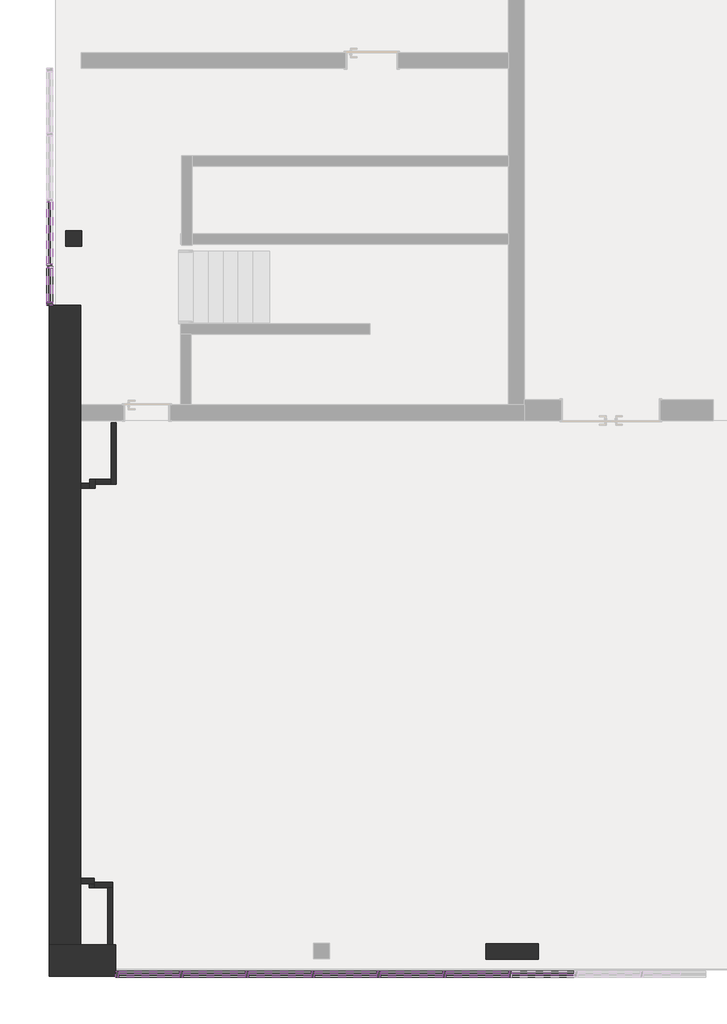
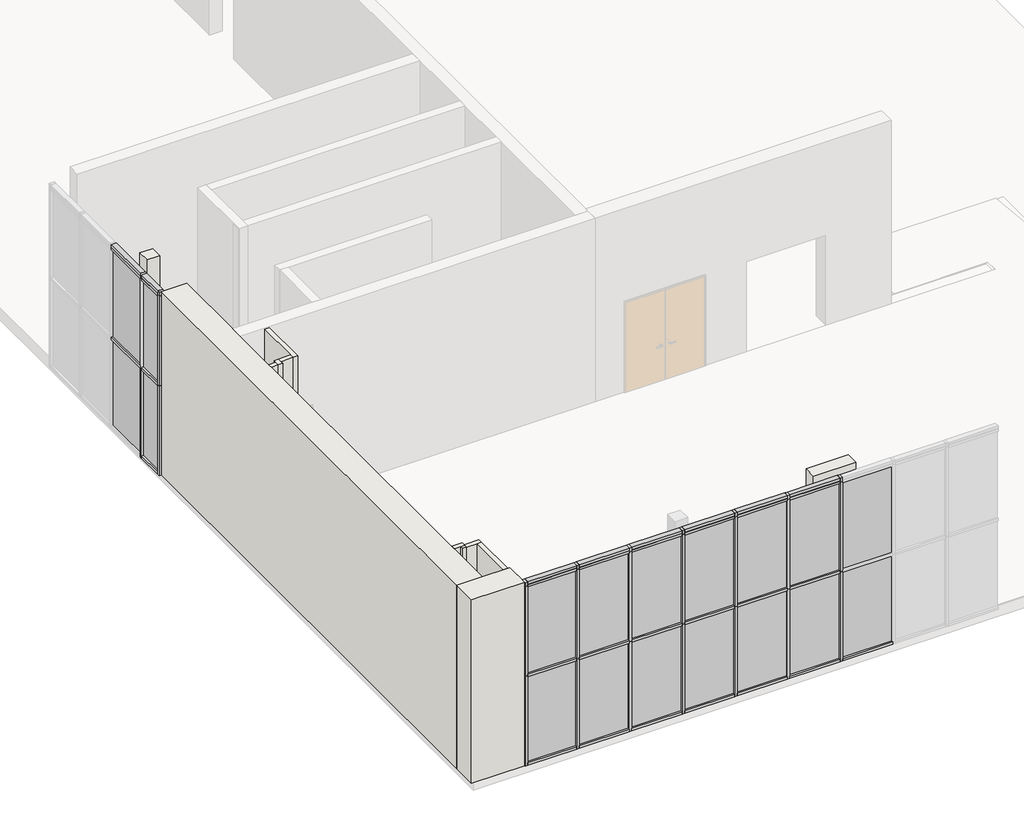
# One storey, part 1 of 5: 57 members, 27 plates, 12 walls.
# Revit data of these elements (continued)
# Elements 1, 2, 3, 4, 5, 6, 7, 8, 9, 10, 11, 12, 13, 14, 15, 16, 17, 18, 19, 20, 21, 22, 23, 24, 25, 26, 27, 28, 29, 30, 31, 32, 33, 34, 35, 36, 37, 38, 39, 40, 41, 42, 43, 44, 45, 46, 47, 48, 49, 50, 51, 52, 53, 54, 55, 56, 57 (IfcMember, "Pfosten rechteckig : 6 x 12")
#   Phase Created = Phase 1
#   Materials on its faces: "Metall - verzinkt"
# Elements 58, 59, 60, 61, 62, 63, 64, 65, 66, 67, 68, 69, 70, 71, 72, 73, 74, 75, 76, 77, 78, 79, 80, 81, 82, 83, 84 (IfcPlate, "Systemelement : Verglasung")
#   Phase Created = Phase 1
#   Materials on its faces: "Glas"
# Element 85 (IfcWall, "STB 30.0 - Sichtbeton 1")
#   Comments = ""
#   Top Offset = 0.000 m
#   Base Offset = 0.000 m
#   wall height = 4.600 m
#   Phase Created = Phase 1
#   Base Constraint = EFH
#   Top Constraint = UK Decke EG
#   Materials on its faces: "Stahlbeton - Sichtbeton (1)"
# Elements 86, 87, 88, 89, 90, 91, 92 (IfcWall, "GK 10.0")
#   Top Offset = 0.000 m
#   Base Offset = 0.000 m
#   wall height = 4.600 m
#   Phase Created = Phase 1
#   Base Constraint = EFH
#   Top Constraint = UK Decke EG
#   Materials on its faces: "Gipswandbauplatte"
# Element 93 (IfcWall, "GK 10.0 grau")
#   Top Offset = 0.000 m
#   Base Offset = 0.000 m
#   wall height = 4.600 m
#   Phase Created = Phase 1
#   Base Constraint = EFH
#   Top Constraint = UK Decke EG
#   Materials on its faces: "Gipswandbauplatte"
# Element 94 (IfcWall, "STB 30.0")
#   Comments = ""
#   Top Offset = 0.000 m
#   Base Offset = 0.000 m
#   wall height = 4.600 m
#   Phase Created = Phase 1
#   Base Constraint = EFH
#   Top Constraint = UK Decke EG
#   Materials on its faces: "Stahlbeton - Ortbeton"
# Element 95 (IfcWall, "STB 48 schwarz")
#   Comments = ""
#   Top Offset = 0.000 m
#   Base Offset = 0.000 m
#   wall height = 4.600 m
#   Phase Created = Phase 1
#   Base Constraint = EFH
#   Top Constraint = UK Decke EG
#   Materials on its faces: "Vorgabe - Wand", "Kunststoff - Grau", "Wärmedämmung - hart"
# Element 96 (IfcWall, "STB 48.0 WD 12.0")
#   Comments = ""
#   Top Offset = 0.000 m
#   Base Offset = 0.000 m
#   wall height = 4.600 m
#   Phase Created = Phase 1
#   Base Constraint = EFH
#   Top Constraint = UK Decke EG
#   Materials on its faces: "Vorgabe - Wand", "Wärmedämmung - hart", "Stahlbeton - Ortbeton"
# Materials
#   "Stahlbeton - Sichtbeton (1)": class "Beton", colour RGB 192 192 192, transparency 0, Cost = 0
#   "Gipswandbauplatte": class "Allgemeines", colour RGB 0 0 0, transparency 0, Description = "Gipswandbauplatte", Cost = 0
#   "Wärmedämmung - hart": class "Stuck", colour RGB 255 255 255, transparency 0, Description = "Äußere Oberfläche", Cost = 0
#   "Stahlbeton - Ortbeton": class "Beton", colour RGB 247 247 247, transparency 0, Cost = 0
#   "Kunststoff - Grau": class "Kunststoff", colour RGB 0 0 0, transparency 0, Cost = 0
#   "Metall - verzinkt": class "Allgemeines", colour RGB 200 200 200, transparency 0, Cost = 0
#   "Glas": class "Glas", colour RGB 0 0 255, transparency 0.75, Comments = "Render-Darstellung nicht aktualisiert ", Cost = 0
#   "Vorgabe - Wand": class "Stuck", colour RGB 128 128 128, transparency 0, Description = "Äußere Oberfläche", Cost = 0
